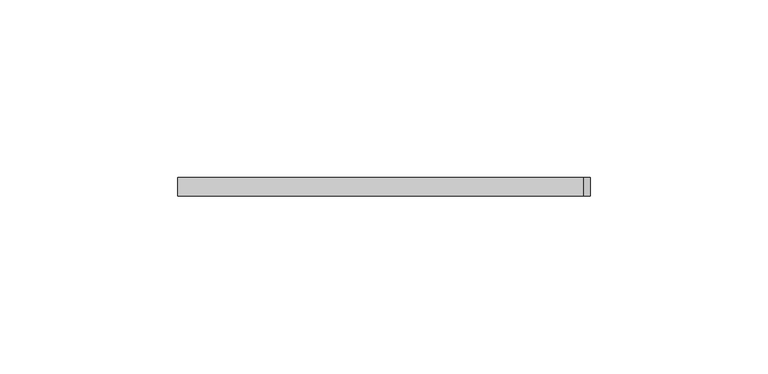
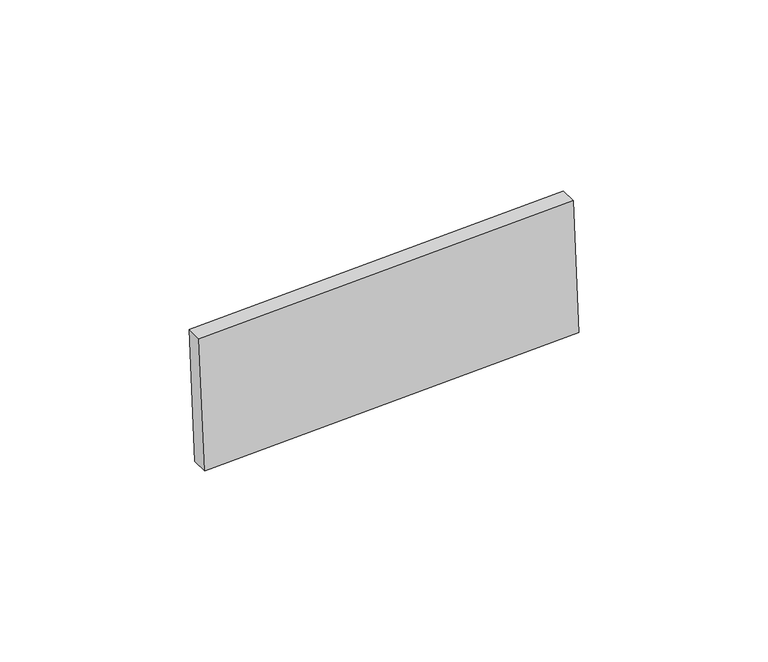
"""IFC4 building model written with IfcOpenShell, lengths in millimetres: proxy geometry, Inner panel:Inner panel:1:Inner panel:1 : Inner panel:Inner panel:300324:2:Inner panel:1:Inner panel:1 : Inner panel:Inner panel:300324:2 : Inner panel:Inner panel:1:Inner panel:1 : Inner panel:Inner panel:300324:300043:168 : Inner panel:Inner panel:1:Inner panel:1 : Inner panel:Inner panel:300324:2:Inner panel:1:Inner panel:1 : Inner panel:Inner panel:300324:2 : Inner panel:Inner panel:1:Inner panel:1 : Inner panel:Inner panel:300324:300043:308120."""

from ifc_helpers import new_model, si_unit, frame, origin, place, context, project, spatial, polyline, outline, extrude, source, transform, mapped, element, save


def generic_models_5e04cdec(model_context):
    return source(origin(), model_context, "Body", "SweptSolid", [
        extrude(outline(polyline([(0.0, -114.3), (0.0, 0.0), (5.213809, 0.0), (5.213809, -114.3), (0.0, -114.3)])), frame((560425.2415304, -565806.907991, 3954.8593665), z_axis=(-0.04163054471216399, 0.0, 0.9991330730923527), x_axis=(0.0, -1.0, 0.0)), (0.0, 0.0, 1.0), 43.2233908),
    ])


if __name__ == "__main__":
    model = new_model("IFC4")
    model_context = context("Model", 3, world=origin())
    ifc_project = project(units=[si_unit("LENGTHUNIT", "METRE", prefix="MILLI")], contexts=[model_context])
    site = spatial("IfcSite", under=ifc_project)
    building = spatial("IfcBuilding", under=site)
    placement = place(None, origin())
    generic_models_shape = generic_models_5e04cdec(model_context)
    element("IfcBuildingElementProxy", 1, Name="Inner panel:Inner panel:1:Inner panel:1 : Inner panel:Inner panel:300324:2:Inner panel:1:Inner panel:1 : Inner panel:Inner panel:300324:2 : Inner panel:Inner panel:1:Inner panel:1 : Inner panel:Inner panel:300324:300043:168 : Inner panel:Inner panel:1:Inner panel:1 : Inner panel:Inner panel:300324:2:Inner panel:1:Inner panel:1 : Inner panel:Inner panel:300324:2 : Inner panel:Inner panel:1:Inner panel:1 : Inner panel:Inner panel:300324:300043:308120", ObjectType="Inner panel:Inner panel:1:Inner panel:1 : Inner panel:Inner panel:300324:2:Inner panel:1:Inner panel:1 : Inner panel:Inner panel:300324:2 : Inner panel:Inner panel:1:Inner panel:1 : Inner panel:Inner panel:300324:300043:168 : Inner panel:Inner panel:1:Inner panel:1 : Inner panel:Inner panel:300324:2:Inner panel:1:Inner panel:1 : Inner panel:Inner panel:300324:2 : Inner panel:Inner panel:1:Inner panel:1 : Inner panel:Inner panel:300324:300043:308120", at=placement, inside=building, context=model_context, shape_type="MappedRepresentation", body=[
        mapped(generic_models_shape, transform((0.0, 0.0, 0.0), x_axis=(1.0, 0.0, 0.0), y_axis=(0.0, 1.0, 0.0), z_axis=(0.0, 0.0, 1.0))),
    ])
    save(model, "model.ifc")

# Revit data of these elements
# Type "Inner panel:Inner panel:1:Inner panel:1 : Inner panel:Inner panel:300324:2:Inner panel:1:Inner panel:1 : Inner panel:Inner panel:300324:2 : Inner panel:Inner panel:1:Inner panel:1 : Inner panel:Inner panel:300324:300043:168 : Inner panel:Inner panel:1:Inner panel:1 : Inner panel:Inner panel:300324:2:Inner panel:1:Inner panel:1 : Inner panel:Inner panel:300324:2 : Inner panel:Inner panel:1:Inner panel:1 : Inner panel:Inner panel:300324:300043:308120"
#   NameOverride = "Inner panel:Inner panel:1:Inner panel:1 : Inner panel:Inner panel:300324:2:Inner panel:1:Inner panel:1 : Inner panel:Inner panel:300324:2 : Inner panel:Inner panel:1:Inner panel:1 : Inner panel:Inner panel:300324:300043:308120"
#   ObjectTypeOverride = "Inner panel:1:Inner panel:1 : Inner panel:Inner panel:300324:2 : Inner panel:Inner panel:1:Inner panel:1 : Inner panel:Inner panel:300324:300043"
#   Reference = "Inner panel"
#   Tag = "308120"
# Element 1 (IfcBuildingElementProxy, "Inner panel:Inner panel:1:Inner panel:1 : Inner panel:Inner panel:300324:2:Inner panel:1:Inner panel:1 : Inner panel:Inner panel:300324:2 : Inner panel:Inner panel:1:Inner panel:1 : Inner panel:Inner panel:300324:300043:168 : Inner panel:Inner panel:1:Inner panel:1 : Inner panel:Inner panel:300324:2:Inner panel:1:Inner panel:1 : Inner panel:Inner panel:300324:2 : Inner panel:Inner panel:1:Inner panel:1 : Inner panel:Inner panel:300324:300043:308120")
#   Materials on its faces: "SLIDING CLIP"
# Materials
#   "SLIDING CLIP": class "Generic", colour RGB 120 120 120, transparency 0, Cost = 0
